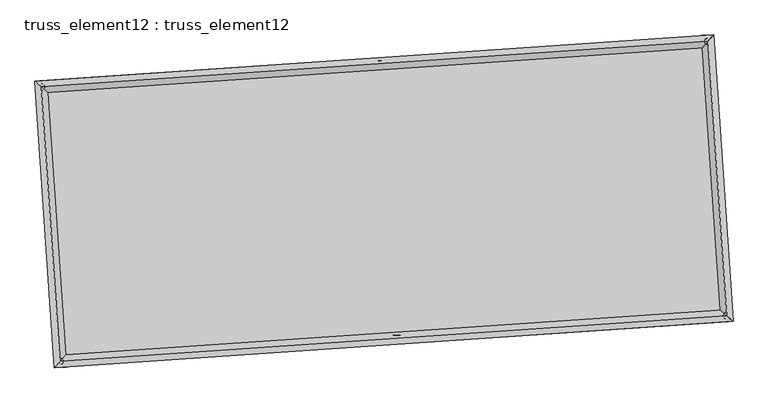
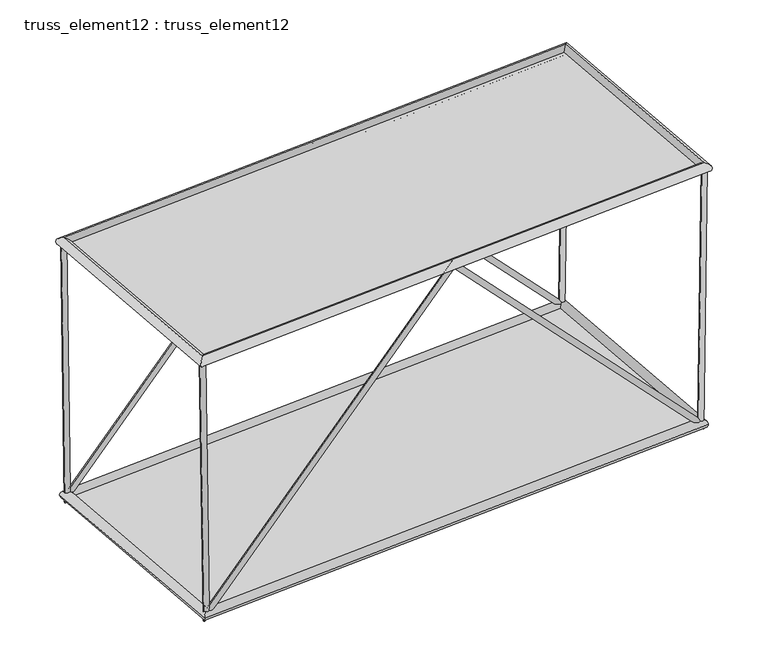
"""IFC4 building model written with IfcOpenShell, lengths in millimetres: plate geometry, truss_element12 : truss_element12."""

from ifc_helpers import new_model, si_unit, frame, origin, origin_with_axes, place, context, project, spatial, polyline, circle_curve, ellipse_curve, outline, extrude, source, transform, mapped, element, save
from ifc_brep_helpers import plane_surface, cylinder_surface, advanced_brep


def truss_element12_truss_element12_96d65a0f(model_context):
    return source(origin(), model_context, "Body", "SolidModel", [
        advanced_brep(
        [(-3734.3431589, 2271.4917397, 5000.2102148), (-3833.4368926, 2258.1311618, 4998.822083), (-3666.6361351, 2276.1084243, 122.4145391), (-3762.3507477, 2262.9782558, -122.4145391), (1064.352803, 2598.6965758, 5071.6275538), (1064.7915465, 2592.1227392, 4927.3870518), (5794.1054726, 2921.2004309, 122.4057644), (5890.6555044, 2921.1800576, -122.4057644), (5863.0394836, 2925.9007791, 5000.2050975), (5963.0292669, 2926.1149494, 4998.791816)],
        [
            (0, 1, circle_curve(frame((-3783.8900257, 2264.8114508, 4999.5161489), z_axis=(-0.013879316866172189, -0.0009463778568816287, 0.9999032297839028), x_axis=(-0.13360598716352348, 0.9910341064360698, -0.0009165557926168256)), 50.0)),
            (1, 0, circle_curve(frame((-3783.8900257, 2264.8114508, 4999.5161489), z_axis=(-0.013879316866172189, -0.0009463778568816287, 0.9999032297839028), x_axis=(-0.13360598716352348, 0.9910341064360698, -0.0009165557926168256)), 50.0)),
            (0, 2),
            (2, 3, ellipse_curve(frame((-3714.4934414, 2269.54334, 0.0), z_axis=(-0.9283327861344515, -0.06329948376321365, 0.36632146202912724), x_axis=(0.3654728402923336, 0.0249202036872039, 0.9304883591194695)), 131.8459204, 50.0)),
            (3, 1),
            (3, 2, ellipse_curve(frame((-3714.4934414, 2269.54334, 0.0), z_axis=(-0.9283327861344515, -0.06329948376321365, 0.36632146202912724), x_axis=(0.3654728402923336, 0.0249202036872039, 0.9304883591194695)), 131.8459204, 50.0)),
            (2, 4),
            (4, 5, ellipse_curve(frame((1064.5721747, 2595.4096575, 4999.5073028), z_axis=(-0.997683393920353, -0.06802823808179366, 6.571949967902977e-05), x_axis=(-6.556725362809862e-05, -4.47078178024543e-06, -0.9999999978404737)), 72.2772914, 50.0)),
            (5, 3),
            (5, 4, ellipse_curve(frame((1064.5721747, 2595.4096575, 4999.5073028), z_axis=(-0.997683393920353, -0.06802823808179366, 6.571949967902977e-05), x_axis=(-6.556725362809862e-05, -4.47078178024543e-06, -0.9999999978404737)), 72.2772914, 50.0)),
            (4, 6),
            (6, 7, ellipse_curve(frame((5842.3804885, 2921.1902443, 0.0), z_axis=(-0.9284028499826135, -0.06330426115068234, -0.3661430303369535), x_axis=(-0.36529482195571816, -0.024908065293541393, 0.9305585856546985)), 131.8265203, 50.0)),
            (7, 5),
            (7, 6, ellipse_curve(frame((5842.3804885, 2921.1902443, 0.0), z_axis=(-0.9284028499826135, -0.06330426115068234, -0.3661430303369535), x_axis=(-0.36529482195571816, -0.024908065293541393, 0.9305585856546985)), 131.8265203, 50.0)),
            (8, 9, circle_curve(frame((5913.0343752, 2926.0078642, 4999.4984567), z_axis=(0.014130777343731374, 0.000963523990955459, 0.9998996913456772), x_axis=(-0.0021551055619355025, 0.9999972423609006, -0.0009331616212425731)), 50.0)),
            (9, 8, circle_curve(frame((5913.0343752, 2926.0078642, 4999.4984567), z_axis=(0.014130777343731374, 0.000963523990955459, 0.9998996913456772), x_axis=(-0.0021551055619355025, 0.9999972423609006, -0.0009331616212425731)), 50.0)),
            (6, 8),
            (9, 7),
        ],
        [
            plane_surface(frame((-3783.8900257, 2314.8114284, 4999.5634724), z_axis=(-0.013879316866172062, -0.0009463778568853915, 0.9999032297839029), x_axis=(0.999903677642666, -1.3136343474329246e-05, 0.013879310649599583))),
            cylinder_surface(frame((-3783.8900257, 2264.8114508, 4999.5161489), z_axis=(-0.013879316866172192, -0.0009463778568816289, 0.999903229783903), x_axis=(-0.13360598716352348, 0.9910341064360698, -0.0009165557926168256)), 50.0),
            cylinder_surface(frame((-3714.4934414, 2269.54334, 0.0), z_axis=(-0.690224976549348, -0.04706381736012723, -0.7220626557598343), x_axis=(-0.02041786679877859, 0.998751974095415, -0.04558075203305543)), 50.0),
            cylinder_surface(frame((1064.5721747, 2595.4096575, 4999.5073028), z_axis=(-0.6901302832567453, -0.047057360584467835, 0.7221535826586948), x_axis=(-0.11534897013780812, 0.9922789830256344, -0.045574498721981514)), 50.0),
            plane_surface(frame((5913.0343752, 2876.0078874, 4999.5466377), z_axis=(0.014130777343731945, 0.000963523990955734, 0.9998996913456772), x_axis=(0.999900155581377, -1.3616702533525447e-05, -0.014130770783065592))),
            cylinder_surface(frame((5842.3804885, 2921.1902443, 0.0), z_axis=(-0.014130777343731377, -0.0009635239909554592, -0.9998996913456775), x_axis=(-0.0021551055619355025, 0.9999972423609006, -0.0009331616212425731)), 50.0),
        ],
        [
            (0, [[1, 2]]),
            (1, [[-1, 3, 4, 5]]),
            (1, [[-2, -5, 6, -3]]),
            (2, [[-4, 7, 8, 9]]),
            (2, [[-6, -9, 10, -7]]),
            (3, [[-8, 11, 12, 13]]),
            (3, [[-10, -13, 14, -11]]),
            (4, [[15, 16]]),
            (5, [[-12, 17, -16, 18]]),
            (5, [[-14, -18, -15, -17]]),
        ],
    ),
        advanced_brep(
        [(-3462.230206, -1719.2418446, 5000.2102148), (-3561.3239397, -1732.6024225, 4998.822083), (-3394.5231822, -1714.62516, 122.4145391), (-3490.2377948, -1727.7553285, -122.4145391), (1336.4657559, -1392.0370085, 5071.6275538), (1336.9044994, -1398.6108451, 4927.3870518), (6066.2184255, -1069.5331534, 122.4057644), (6162.7684573, -1069.5535267, -122.4057644), (6135.1524365, -1064.8328052, 5000.2050975), (6235.1422198, -1064.6186349, 4998.791816)],
        [
            (0, 1, circle_curve(frame((-3511.7770728, -1725.9221335, 4999.5161489), z_axis=(-0.013879316866172014, -0.000946377856881616, 0.9999032297839029), x_axis=(-0.1336059871635238, 0.9910341064360699, -0.0009165557926168189)), 50.0)),
            (1, 0, circle_curve(frame((-3511.7770728, -1725.9221335, 4999.5161489), z_axis=(-0.013879316866172014, -0.000946377856881616, 0.9999032297839029), x_axis=(-0.1336059871635238, 0.9910341064360699, -0.0009165557926168189)), 50.0)),
            (0, 2),
            (2, 3, ellipse_curve(frame((-3442.3804885, -1721.1902443, 0.0), z_axis=(-0.9283327861344514, -0.06329948376321375, 0.3663214620291273), x_axis=(0.3654728402923336, 0.02492020368720394, 0.9304883591194695)), 131.8459204, 50.0)),
            (3, 1),
            (3, 2, ellipse_curve(frame((-3442.3804885, -1721.1902443, 0.0), z_axis=(-0.9283327861344514, -0.06329948376321375, 0.3663214620291273), x_axis=(0.3654728402923336, 0.02492020368720394, 0.9304883591194695)), 131.8459204, 50.0)),
            (2, 4),
            (4, 5, ellipse_curve(frame((1336.6851277, -1395.3239268, 4999.5073028), z_axis=(-0.997683393920353, -0.06802823808179373, 6.571949967870881e-05), x_axis=(-6.556725362779111e-05, -4.470781780274258e-06, -0.9999999978404737)), 72.2772914, 50.0)),
            (5, 3),
            (5, 4, ellipse_curve(frame((1336.6851277, -1395.3239268, 4999.5073028), z_axis=(-0.997683393920353, -0.06802823808179373, 6.571949967870881e-05), x_axis=(-6.556725362779111e-05, -4.470781780274258e-06, -0.9999999978404737)), 72.2772914, 50.0)),
            (4, 6),
            (6, 7, ellipse_curve(frame((6114.4934414, -1069.54334, 0.0), z_axis=(-0.9284028499826134, -0.06330426115068227, -0.3661430303369539), x_axis=(-0.36529482195571855, -0.024908065293541462, 0.9305585856546982)), 131.8265203, 50.0)),
            (7, 5),
            (7, 6, ellipse_curve(frame((6114.4934414, -1069.54334, 0.0), z_axis=(-0.9284028499826134, -0.06330426115068227, -0.3661430303369539), x_axis=(-0.36529482195571855, -0.024908065293541462, 0.9305585856546982)), 131.8265203, 50.0)),
            (8, 9, circle_curve(frame((6185.1473281, -1064.7257201, 4999.4984567), z_axis=(0.014130777343731101, 0.0009635239909553769, 0.9998996913456774), x_axis=(-0.0021551055619351343, 0.9999972423609005, -0.0009331616212424965)), 50.0)),
            (9, 8, circle_curve(frame((6185.1473281, -1064.7257201, 4999.4984567), z_axis=(0.014130777343731101, 0.0009635239909553769, 0.9998996913456774), x_axis=(-0.0021551055619351343, 0.9999972423609005, -0.0009331616212424965)), 50.0)),
            (6, 8),
            (9, 7),
        ],
        [
            plane_surface(frame((-3511.7770728, -1675.9221559, 4999.5634724), z_axis=(-0.013879316866172062, -0.0009463778568853786, 0.9999032297839029), x_axis=(0.999903677642666, -1.3136343474329246e-05, 0.013879310649599583))),
            cylinder_surface(frame((-3511.7770728, -1725.9221335, 4999.5161489), z_axis=(-0.013879316866172014, -0.000946377856881616, 0.9999032297839029), x_axis=(-0.1336059871635238, 0.9910341064360699, -0.0009165557926168189)), 50.0),
            cylinder_surface(frame((-3442.3804885, -1721.1902443, 0.0), z_axis=(-0.6902249765493476, -0.047063817360127276, -0.7220626557598344), x_axis=(-0.02041786679877854, 0.9987519740954149, -0.04558075203305555)), 50.0),
            cylinder_surface(frame((1336.6851277, -1395.3239268, 4999.5073028), z_axis=(-0.6901302832567454, -0.047057360584467856, 0.7221535826586944), x_axis=(-0.11534897013780826, 0.9922789830256344, -0.04557449872198166)), 50.0),
            plane_surface(frame((6185.1473281, -1114.7256969, 4999.5466377), z_axis=(0.014130777343731945, 0.0009635239909557223, 0.9998996913456772), x_axis=(0.999900155581377, -1.3616702533081358e-05, -0.014130770783065592))),
            cylinder_surface(frame((6114.4934414, -1069.54334, 0.0), z_axis=(-0.014130777343731101, -0.0009635239909553769, -0.9998996913456774), x_axis=(-0.0021551055619351343, 0.9999972423609005, -0.0009331616212424965)), 50.0),
        ],
        [
            (0, [[1, 2]]),
            (1, [[-1, 3, 4, 5]]),
            (1, [[-2, -5, 6, -3]]),
            (2, [[-4, 7, 8, 9]]),
            (2, [[-6, -9, 10, -7]]),
            (3, [[-8, 11, 12, 13]]),
            (3, [[-10, -13, 14, -11]]),
            (4, [[15, 16]]),
            (5, [[-12, 17, -16, 18]]),
            (5, [[-14, -18, -15, -17]]),
        ],
    ),
        advanced_brep(
        [(-3511.7817087, -1725.9272716, 4909.5161491), (-3511.772437, -1725.9169954, 5089.5161488), (-3783.8847353, 2264.8069895, 5089.5161488), (-3783.8953162, 2264.815912, 4909.5161491), (5913.0300663, 2926.0027484, 5089.4984566), (5913.0386842, 2926.01298, 4909.4984568), (6185.1423646, -1064.7212365, 5089.4984566), (6185.1522916, -1064.7302037, 4909.4984568)],
        [
            (0, 1, ellipse_curve(frame((-3511.7770728, -1725.9221335, 4999.5161489), z_axis=(-0.7535719234042888, 0.6573654662781608, 1.2871387313806292e-06), x_axis=(-0.6573654662769124, -0.7535719234053778, 1.2871387313806982e-06)), 127.2792206, 90.0)),
            (1, 2),
            (2, 3, ellipse_curve(frame((-3783.8900257, 2264.8114508, 4999.5161489), z_axis=(-0.6573654662769123, -0.753571923405378, 1.2871387313807605e-06), x_axis=(0.753571923404289, -0.6573654662781606, -1.2871387313806917e-06)), 127.2792206, 90.0)),
            (3, 0),
            (1, 0, ellipse_curve(frame((-3511.7770728, -1725.9221335, 4999.5161489), z_axis=(-0.7535719234042888, 0.6573654662781608, 1.2871387313806292e-06), x_axis=(-0.6573654662769124, -0.7535719234053778, 1.2871387313806982e-06)), 127.2792206, 90.0)),
            (3, 2, ellipse_curve(frame((-3783.8900257, 2264.8114508, 4999.5161489), z_axis=(-0.6573654662769123, -0.753571923405378, 1.2871387313807605e-06), x_axis=(0.753571923404289, -0.6573654662781606, -1.2871387313806917e-06)), 127.2792206, 90.0)),
            (2, 4),
            (4, 5, ellipse_curve(frame((5913.0343752, 2926.0078642, 4999.4984567), z_axis=(-0.7535719234042888, 0.6573654662781608, 1.2871387313807556e-06), x_axis=(-0.6573654662769126, -0.7535719234053777, 1.2871387313806968e-06)), 127.2792206, 90.0)),
            (5, 3),
            (5, 4, ellipse_curve(frame((5913.0343752, 2926.0078642, 4999.4984567), z_axis=(-0.7535719234042888, 0.6573654662781608, 1.2871387313807556e-06), x_axis=(-0.6573654662769126, -0.7535719234053777, 1.2871387313806968e-06)), 127.2792206, 90.0)),
            (4, 6),
            (6, 7, ellipse_curve(frame((6185.1473281, -1064.7257201, 4999.4984567), z_axis=(0.6573654662769123, 0.753571923405378, -1.287138731380634e-06), x_axis=(-0.7535719234042889, 0.6573654662781607, 1.2871387313806936e-06)), 127.2792206, 90.0)),
            (7, 5),
            (7, 6, ellipse_curve(frame((6185.1473281, -1064.7257201, 4999.4984567), z_axis=(0.6573654662769123, 0.753571923405378, -1.287138731380634e-06), x_axis=(-0.7535719234042889, 0.6573654662781607, 1.2871387313806936e-06)), 127.2792206, 90.0)),
            (6, 1),
            (0, 7),
        ],
        [
            cylinder_surface(frame((-3511.7770728, -1725.9221335, 4999.5161489), z_axis=(0.0680282382287011, -0.9976833960748768, 0.0), x_axis=(-0.9976833945508086, -0.06802823812478068, 5.5273991576084965e-05)), 90.0),
            cylinder_surface(frame((-3783.8900257, 2264.8114508, 4999.5161489), z_axis=(-0.9976833960732239, -0.06802823822858783, 1.8202890505743231e-06), x_axis=(-0.06802823803443628, 0.9976833946561564, 5.3453702528111224e-05)), 90.0),
            cylinder_surface(frame((5913.0343752, 2926.0078642, 4999.4984567), z_axis=(-0.06802823822870105, 0.9976833960748767, 0.0), x_axis=(0.9976833947449599, 0.06802823813801909, 5.1633413480137484e-05)), 90.0),
            cylinder_surface(frame((6185.1473281, -1064.7257201, 4999.4984567), z_axis=(0.9976833960732238, 0.068028238228588, -1.820289050574235e-06), x_axis=(0.068028238228588, -0.9976833946429179, 5.345370252811124e-05)), 90.0),
        ],
        [
            (0, [[1, 2, 3, 4]]),
            (0, [[5, -4, 6, -2]]),
            (1, [[-3, 7, 8, 9]]),
            (1, [[-6, -9, 10, -7]]),
            (2, [[-8, 11, 12, 13]]),
            (2, [[-10, -13, 14, -11]]),
            (3, [[-12, 15, -1, 16]]),
            (3, [[-14, -16, -5, -15]]),
        ],
    ),
        advanced_brep(
        [(-3358.7115243, -1625.2761972, 0.0), (-3526.0494527, -1817.1042913, 0.0), (-3810.4074885, 2353.2123043, 0.0), (-3618.5793943, 2185.8743758, 0.0), (5926.0494527, 3017.1042913, 0.0), (5758.7115243, 2825.2761972, 0.0), (6210.4074885, -1153.2123043, 0.0), (6018.5793943, -985.8743758, 0.0)],
        [
            (0, 1, ellipse_curve(frame((-3442.3804885, -1721.1902443, 0.0), z_axis=(-0.753571923405459, 0.6573654662780796, 0.0), x_axis=(-0.6573654662780797, -0.753571923405459, 0.0)), 127.2792206, 90.0)),
            (1, 2),
            (2, 3, ellipse_curve(frame((-3714.4934414, 2269.54334, 0.0), z_axis=(-0.6573654662780796, -0.7535719234054591, 0.0), x_axis=(0.7535719234054591, -0.6573654662780796, 0.0)), 127.2792206, 90.0)),
            (3, 0),
            (1, 0, ellipse_curve(frame((-3442.3804885, -1721.1902443, 0.0), z_axis=(-0.753571923405459, 0.6573654662780796, 0.0), x_axis=(-0.6573654662780797, -0.753571923405459, 0.0)), 127.2792206, 90.0)),
            (3, 2, ellipse_curve(frame((-3714.4934414, 2269.54334, 0.0), z_axis=(-0.6573654662780796, -0.7535719234054591, 0.0), x_axis=(0.7535719234054591, -0.6573654662780796, 0.0)), 127.2792206, 90.0)),
            (2, 4),
            (4, 5, ellipse_curve(frame((5842.3804885, 2921.1902443, 0.0), z_axis=(-0.753571923405459, 0.6573654662780796, 0.0), x_axis=(-0.6573654662780797, -0.7535719234054589, 0.0)), 127.2792206, 90.0)),
            (5, 3),
            (5, 4, ellipse_curve(frame((5842.3804885, 2921.1902443, 0.0), z_axis=(-0.753571923405459, 0.6573654662780796, 0.0), x_axis=(-0.6573654662780797, -0.7535719234054589, 0.0)), 127.2792206, 90.0)),
            (4, 6),
            (6, 7, ellipse_curve(frame((6114.4934414, -1069.54334, 0.0), z_axis=(0.6573654662780796, 0.7535719234054589, 0.0), x_axis=(-0.7535719234054589, 0.6573654662780799, 0.0)), 127.2792206, 90.0)),
            (7, 5),
            (7, 6, ellipse_curve(frame((6114.4934414, -1069.54334, 0.0), z_axis=(0.6573654662780796, 0.7535719234054589, 0.0), x_axis=(-0.7535719234054589, 0.6573654662780799, 0.0)), 127.2792206, 90.0)),
            (6, 1),
            (0, 7),
        ],
        [
            cylinder_surface(frame((-3442.3804885, -1721.1902443, 0.0), z_axis=(0.06802823822870319, -0.9976833960748764, 0.0), x_axis=(-0.9976833960748764, -0.06802823822870319, 0.0)), 90.0),
            cylinder_surface(frame((-3714.4934414, 2269.54334, 0.0), z_axis=(-0.9976833960748764, -0.06802823822870263, 0.0), x_axis=(-0.06802823822870263, 0.9976833960748764, 0.0)), 90.0),
            cylinder_surface(frame((5842.3804885, 2921.1902443, 0.0), z_axis=(-0.06802823822870303, 0.9976833960748764, 0.0), x_axis=(0.9976833960748764, 0.06802823822870303, 0.0)), 90.0),
            cylinder_surface(frame((6114.4934414, -1069.54334, 0.0), z_axis=(0.9976833960748767, 0.06802823822870256, 0.0), x_axis=(0.06802823822870256, -0.9976833960748767, 0.0)), 90.0),
        ],
        [
            (0, [[1, 2, 3, 4]]),
            (0, [[5, -4, 6, -2]]),
            (1, [[-3, 7, 8, 9]]),
            (1, [[-6, -9, 10, -7]]),
            (2, [[-8, 11, 12, 13]]),
            (2, [[-10, -13, 14, -11]]),
            (3, [[-12, 15, -1, 16]]),
            (3, [[-14, -16, -5, -15]]),
        ],
    ),
        extrude(outline(polyline([(-3442.3804885, -1721.1902443), (-3714.4934414, 2269.54334), (5842.3804885, 2921.1902443), (6114.4934414, -1069.54334), (-3442.3804885, -1721.1902443)])), origin_with_axes(), (0.0, 0.0, 1.0), 20.0),
        extrude(outline(polyline([(-1999.9999999, 4859.7202475), (2000.0000001, 4859.7202474), (2000.0, -4859.7202475), (-2000.0, -4859.7202475), (-1999.9999999, 4859.7202475)])), frame((1200.6286512, 600.0428653, 4999.5073028), z_axis=(1.81607216181486e-06, 1.2383105717756673e-07, 0.9999999999983434), x_axis=(-0.06802823822870303, 0.9976833960748765, 0.0)), (0.0, 0.0, 1.0), 20.0),
    ])


if __name__ == "__main__":
    model = new_model("IFC4")
    model_context = context("Model", 3, world=origin())
    ifc_project = project(units=[si_unit("LENGTHUNIT", "METRE", prefix="MILLI")], contexts=[model_context])
    site = spatial("IfcSite", under=ifc_project)
    building = spatial("IfcBuilding", under=site)
    placement = place(None, origin())
    truss_element12_truss_element12_shape = truss_element12_truss_element12_96d65a0f(model_context)
    element("IfcPlate", 1, ObjectType="truss_element12 : truss_element12", at=placement, inside=building, context=model_context, shape_type="MappedRepresentation", body=[
        mapped(truss_element12_truss_element12_shape, transform((0.0, 0.0, 0.0), x_axis=(1.0, 0.0, 0.0), y_axis=(0.0, 1.0, 0.0), z_axis=(0.0, 0.0, 1.0))),
    ])
    save(model, "model.ifc")

# Revit data of these elements
# Type "truss_element12 : truss_element12"
#   steellbar1 = 90 mm
#   steelbar2 = 50 mm
#   offset1 = 5000 mm
#   M = Default Roof
# Element 1 (IfcPlate, "truss_element12 : truss_element12")
#   Materials on its faces: "Default Roof"
# Materials
#   "Default Roof": class "Miscellaneous", colour RGB 0 127 0, transparency 0, Comments = "Rendering appearance not upgraded Rendering appearance not upgraded ", Cost = 0
